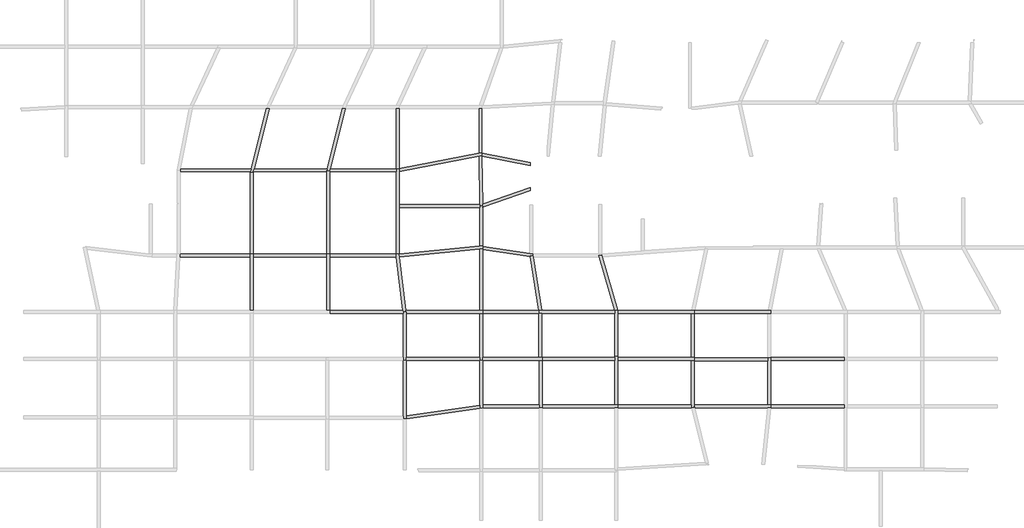
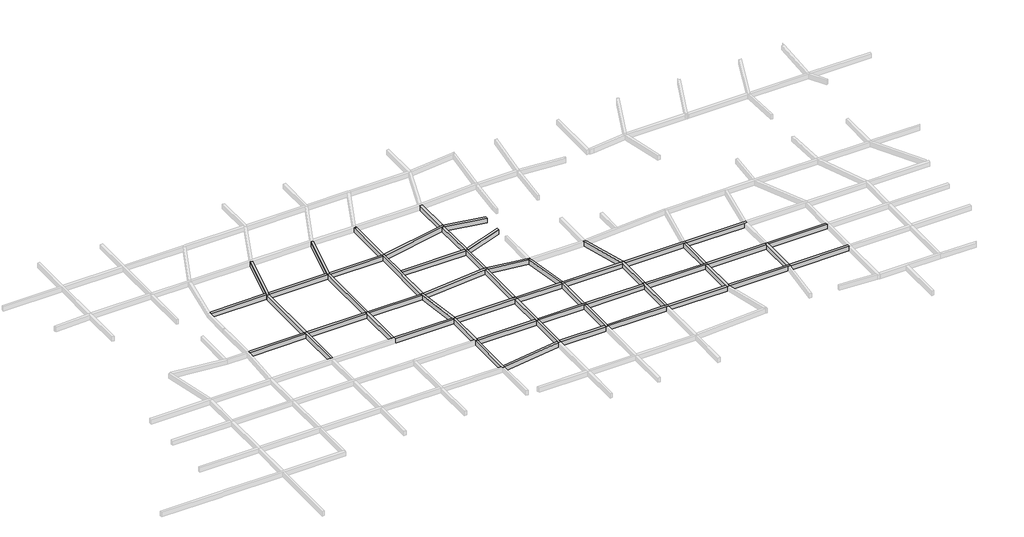
# One storey, part 5 of 15: 56 beams.
"""IFC4 building model written with IfcOpenShell, lengths in millimetres."""

from ifc_helpers import new_model, si_unit, frame, origin, place, context, project, spatial, polyline, outline, extrude, faceted_brep, element, save

model = new_model("IFC4")

# Units and contexts
model_context = context("Model", 3, world=origin())
ifc_project = project(units=[si_unit("LENGTHUNIT", "METRE", prefix="MILLI")], contexts=[model_context])

# Site, building, storey
site = spatial("IfcSite", under=ifc_project)
building = spatial("IfcBuilding", under=site)
storey = spatial("IfcBuildingStorey", under=building, Name="层高", Elevation=3300.0)

# Beams
placement = place(None, origin())
element("IfcBeam", 1, ObjectType="混凝土 - 矩形梁 : KL_beam", at=placement, inside=storey, context=model_context, shape_type="Brep", body=[
    faceted_brep([(196149.7804968, 49107.4754781, 3300.0), (195849.7804968, 49107.4754781, 3300.0), (195849.7804968, 48807.4754781, 3300.0), (195849.7804968, 43342.2492414, 3300.0), (196149.7804968, 43342.2492414, 3300.0), (196149.7804968, 48807.4754781, 3300.0), (196149.7804968, 49107.4754781, 2700.0), (196149.7804968, 43342.2492414, 2700.0), (196149.7804968, 48807.4754781, 2700.0), (195849.7804968, 49107.4754781, 2700.0), (195849.7804968, 43342.2492414, 2700.0), (195849.7804968, 48807.4754781, 2700.0)], [[[0, 1, 2, 3, 4, 5]], [[6, 0, 5, 4, 7, 8]], [[9, 6, 8, 7, 10, 11]], [[1, 9, 11, 10, 3, 2]], [[4, 3, 10, 7]], [[1, 0, 6, 9]]]),
])
element("IfcBeam", 2, ObjectType="混凝土 - 矩形梁 : KL_beam", at=placement, inside=storey, context=model_context, shape_type="Brep", body=[
    faceted_brep([(203965.7079926, 49107.4754781, 3300.0), (203665.7079926, 49107.4754781, 3300.0), (203665.7079926, 48807.4754781, 3300.0), (203665.7079926, 43342.2492414, 3300.0), (203965.7079926, 43342.2492414, 3300.0), (203965.7079926, 48807.4754781, 3300.0), (203965.7079926, 49107.4754781, 2700.0), (203965.7079926, 43342.2492414, 2700.0), (203965.7079926, 48807.4754781, 2700.0), (203665.7079926, 49107.4754781, 2700.0), (203665.7079926, 43342.2492414, 2700.0), (203665.7079926, 48807.4754781, 2700.0)], [[[0, 1, 2, 3, 4, 5]], [[6, 0, 5, 4, 7, 8]], [[9, 6, 8, 7, 10, 11]], [[1, 9, 11, 10, 3, 2]], [[4, 3, 10, 7]], [[1, 0, 6, 9]]]),
])
element("IfcBeam", 3, ObjectType="混凝土 - 矩形梁 : KL_beam", at=placement, inside=storey, context=model_context, shape_type="Brep", body=[
    faceted_brep([(211749.7804968, 43201.435443, 3300.0), (211449.7804968, 43183.086657, 3300.0), (211449.7804968, 43042.2492414, 3300.0), (211449.7804968, 38542.26105, 3300.0), (211449.7804968, 38242.26105, 3300.0), (211749.7804968, 38242.26105, 3300.0), (211749.7804968, 38539.4462664, 3300.0), (211749.7804968, 43039.4462664, 3300.0), (211449.7804968, 43183.086657, 2700.0), (211449.7804968, 43042.2492414, 2700.0), (211449.7804968, 38542.26105, 2700.0), (211449.7804968, 38242.26105, 2700.0), (211749.7804968, 43201.435443, 2700.0), (211749.7804968, 43039.4462664, 2700.0), (211749.7804968, 38539.4462664, 2700.0), (211749.7804968, 38242.26105, 2700.0)], [[[0, 1, 2, 3, 4, 5, 6, 7]], [[1, 8, 9, 10, 11, 4, 3, 2]], [[8, 12, 13, 14, 15, 11, 10, 9]], [[12, 0, 7, 6, 5, 15, 14, 13]], [[5, 4, 11, 15]], [[0, 12, 8, 1]]]),
])
element("IfcBeam", 4, ObjectType="混凝土 - 矩形梁 : KL_beam", at=placement, inside=storey, context=model_context, shape_type="Brep", body=[
    faceted_brep([(211449.7804968, 32262.7548984, 3300.0), (211749.7804968, 32262.7548984, 3300.0), (211749.7804968, 32565.9979708, 3300.0), (211749.7804968, 38239.4462664, 3300.0), (211749.7804968, 38242.26105, 3300.0), (211449.7804968, 38242.26105, 3300.0), (211449.7804968, 32542.26105, 3300.0), (211449.7804968, 32262.7548984, 2700.0), (211449.7804968, 38242.26105, 2700.0), (211449.7804968, 32542.26105, 2700.0), (211749.7804968, 32262.7548984, 2700.0), (211749.7804968, 38242.26105, 2700.0), (211749.7804968, 38239.4462664, 2700.0), (211749.7804968, 32565.9979708, 2700.0)], [[[0, 1, 2, 3, 4, 5, 6]], [[7, 0, 6, 5, 8, 9]], [[10, 7, 9, 8, 11, 12, 13]], [[1, 10, 13, 12, 11, 4, 3, 2]], [[5, 4, 11, 8]], [[1, 0, 7, 10]]]),
])
element("IfcBeam", 5, ObjectType="混凝土 - 矩形梁 : KL_beam", at=placement, inside=storey, context=model_context, shape_type="Brep", body=[
    faceted_brep([(210725.2131667, 49084.2140037, 3300.0), (210759.1923851, 48807.4754781, 3300.0), (211430.2377888, 43342.2492414, 3300.0), (211449.7804968, 43183.086657, 3300.0), (211749.7804968, 43201.435443, 3300.0), (211732.8348985, 43339.4462664, 3300.0), (211059.55045, 48822.9080592, 3300.0), (211022.9770122, 49120.7748067, 3300.0), (211749.7804968, 43201.435443, 2700.0), (211732.8348985, 43339.4462664, 2700.0), (211059.55045, 48822.9080592, 2700.0), (211022.9770122, 49120.7748067, 2700.0), (211449.7804968, 43183.086657, 2700.0), (211430.2377888, 43342.2492414, 2700.0), (210759.1923851, 48807.4754781, 2700.0), (210725.2131667, 49084.2140037, 2700.0)], [[[0, 1, 2, 3, 4, 5, 6, 7]], [[7, 6, 5, 4, 8, 9, 10, 11]], [[11, 10, 9, 8, 12, 13, 14, 15]], [[3, 2, 1, 0, 15, 14, 13, 12]], [[3, 12, 8, 4]], [[0, 7, 11, 15]]]),
])
element("IfcBeam", 6, ObjectType="混凝土 - 矩形梁 : KL_beam", at=placement, inside=storey, context=model_context, shape_type="SweptSolid", body=[
    extrude(outline(polyline([(203965.7079926, 43042.2492414), (203965.7079926, 43342.2492414), (211430.2377888, 43342.2492414), (211449.7804968, 43183.086657), (211449.7804968, 43042.2492414), (203965.7079926, 43042.2492414)])), frame((0.0, 0.0, 2700.0), z_axis=(0.0, 0.0, 1.0), x_axis=(1.0, 0.0, 0.0)), (0.0, 0.0, 1.0), 600.0),
])
element("IfcBeam", 7, ObjectType="混凝土 - 矩形梁 : KL_beam", at=placement, inside=storey, context=model_context, shape_type="Brep", body=[
    faceted_brep([(211732.8348985, 43339.4462664, 3300.0), (211749.7804968, 43201.435443, 3300.0), (211749.7804968, 43042.2492414, 3300.0), (211749.7804968, 43039.4462664, 3300.0), (219249.7804968, 43039.4462664, 3300.0), (219549.7804968, 43039.4462664, 3300.0), (219549.7804968, 43042.26105, 3300.0), (219549.7804968, 43339.4462664, 3300.0), (219249.7804968, 43339.4462664, 3300.0), (211749.7804968, 43039.4462664, 2700.0), (219249.7804968, 43039.4462664, 2700.0), (219549.7804968, 43039.4462664, 2700.0), (211749.7804968, 43201.435443, 2700.0), (211732.8348985, 43339.4462664, 2700.0), (219249.7804968, 43339.4462664, 2700.0), (219549.7804968, 43339.4462664, 2700.0), (219549.7804968, 43042.26105, 2700.0), (211749.7804968, 43042.2492414, 2700.0)], [[[0, 1, 2, 3, 4, 5, 6, 7, 8]], [[3, 9, 10, 11, 5, 4]], [[12, 13, 14, 15, 16, 11, 10, 9, 17]], [[13, 0, 8, 7, 15, 14]], [[9, 3, 2, 1, 12, 17]], [[1, 0, 13, 12]], [[7, 6, 5, 11, 16, 15]]]),
])
element("IfcBeam", 8, ObjectType="混凝土 - 矩形梁 : KL_beam", at=placement, inside=storey, context=model_context, shape_type="Brep", body=[
    faceted_brep([(219249.7804968, 38239.4462664, 3300.0), (219549.7804968, 38239.4462664, 3300.0), (219549.7804968, 38539.4462664, 3300.0), (219549.7804968, 43039.4462664, 3300.0), (219249.7804968, 43039.4462664, 3300.0), (219249.7804968, 38539.4462664, 3300.0), (219249.7804968, 38239.4462664, 2700.0), (219249.7804968, 43039.4462664, 2700.0), (219249.7804968, 38539.4462664, 2700.0), (219549.7804968, 38239.4462664, 2700.0), (219549.7804968, 43039.4462664, 2700.0), (219549.7804968, 38539.4462664, 2700.0)], [[[0, 1, 2, 3, 4, 5]], [[6, 0, 5, 4, 7, 8]], [[9, 6, 8, 7, 10, 11]], [[1, 9, 11, 10, 3, 2]], [[4, 3, 10, 7]], [[1, 0, 6, 9]]]),
])
element("IfcBeam", 9, ObjectType="混凝土 - 矩形梁 : KL_beam", at=placement, inside=storey, context=model_context, shape_type="Brep", body=[
    faceted_brep([(211749.7804968, 38539.4462664, 3300.0), (211749.7804968, 38242.26105, 3300.0), (211749.7804968, 38239.4462664, 3300.0), (219249.7804968, 38239.4462664, 3300.0), (219249.7804968, 38539.4462664, 3300.0), (211749.7804968, 38539.4462664, 2700.0), (219249.7804968, 38539.4462664, 2700.0), (211749.7804968, 38239.4462664, 2700.0), (211749.7804968, 38242.26105, 2700.0), (219249.7804968, 38239.4462664, 2700.0)], [[[0, 1, 2, 3, 4]], [[5, 0, 4, 6]], [[7, 8, 5, 6, 9]], [[2, 7, 9, 3]], [[0, 5, 8, 7, 2, 1]], [[4, 3, 9, 6]]]),
])
element("IfcBeam", 10, ObjectType="混凝土 - 矩形梁 : KL_beam", at=placement, inside=storey, context=model_context, shape_type="Brep", body=[
    faceted_brep([(219249.7804968, 33368.5241292, 3300.0), (219549.7804968, 33412.7548984, 3300.0), (219549.7804968, 33692.26105, 3300.0), (219549.7804968, 38239.4462664, 3300.0), (219249.7804968, 38239.4462664, 3300.0), (219249.7804968, 33671.7672016, 3300.0), (219249.7804968, 33368.5241292, 2700.0), (219249.7804968, 38239.4462664, 2700.0), (219249.7804968, 33671.7672016, 2700.0), (219549.7804968, 33412.7548984, 2700.0), (219549.7804968, 38239.4462664, 2700.0), (219549.7804968, 33692.26105, 2700.0)], [[[0, 1, 2, 3, 4, 5]], [[6, 0, 5, 4, 7, 8]], [[9, 6, 8, 7, 10, 11]], [[1, 9, 11, 10, 3, 2]], [[4, 3, 10, 7]], [[1, 0, 6, 9]]]),
])
element("IfcBeam", 11, ObjectType="混凝土 - 矩形梁 : KL_beam", at=placement, inside=storey, context=model_context, shape_type="SweptSolid", body=[
    extrude(outline(polyline([(211749.7804968, 32262.7548984), (211749.7804968, 32565.9979708), (219249.7804968, 33671.7672016), (219249.7804968, 33368.5241292), (211749.7804968, 32262.7548984)])), frame((0.0, 0.0, 2700.0), z_axis=(0.0, 0.0, 1.0), x_axis=(1.0, 0.0, 0.0)), (0.0, 0.0, 1.0), 600.0),
])
element("IfcBeam", 12, ObjectType="混凝土 - 矩形梁 : KL_beam", at=placement, inside=storey, context=model_context, shape_type="Brep", body=[
    faceted_brep([(225649.7804968, 38239.4462664, 3300.0), (225649.7804968, 38539.4462664, 3300.0), (225589.7804968, 38539.4462664, 3300.0), (225289.7804968, 38539.4462664, 3300.0), (219549.7804968, 38539.4462664, 3300.0), (219549.7804968, 38239.4462664, 3300.0), (225349.7804968, 38239.4462664, 3300.0), (225649.7804968, 38239.4462664, 2700.0), (219549.7804968, 38239.4462664, 2700.0), (225349.7804968, 38239.4462664, 2700.0), (225649.7804968, 38539.4462664, 2700.0), (219549.7804968, 38539.4462664, 2700.0), (225289.7804968, 38539.4462664, 2700.0), (225589.7804968, 38539.4462664, 2700.0)], [[[0, 1, 2, 3, 4, 5, 6]], [[7, 0, 6, 5, 8, 9]], [[10, 7, 9, 8, 11, 12, 13]], [[1, 10, 13, 12, 11, 4, 3, 2]], [[5, 4, 11, 8]], [[1, 0, 7, 10]]]),
])
element("IfcBeam", 13, ObjectType="混凝土 - 矩形梁 : KL_beam", at=placement, inside=storey, context=model_context, shape_type="Brep", body=[
    faceted_brep([(225349.7804968, 33392.26105, 3300.0), (225649.7804968, 33392.26105, 3300.0), (225649.7804968, 33692.26105, 3300.0), (225649.7804968, 38239.4462664, 3300.0), (225349.7804968, 38239.4462664, 3300.0), (225349.7804968, 33692.26105, 3300.0), (225349.7804968, 33392.26105, 2700.0), (225349.7804968, 38239.4462664, 2700.0), (225349.7804968, 33692.26105, 2700.0), (225649.7804968, 33392.26105, 2700.0), (225649.7804968, 38239.4462664, 2700.0), (225649.7804968, 33692.26105, 2700.0)], [[[0, 1, 2, 3, 4, 5]], [[6, 0, 5, 4, 7, 8]], [[9, 6, 8, 7, 10, 11]], [[1, 9, 11, 10, 3, 2]], [[4, 3, 10, 7]], [[1, 0, 6, 9]]]),
])
element("IfcBeam", 14, ObjectType="混凝土 - 矩形梁 : KL_beam", at=placement, inside=storey, context=model_context, shape_type="Brep", body=[
    faceted_brep([(219549.7804968, 33692.26105, 3300.0), (219549.7804968, 33412.7548984, 3300.0), (219549.7804968, 33392.26105, 3300.0), (225349.7804968, 33392.26105, 3300.0), (225349.7804968, 33692.26105, 3300.0), (219549.7804968, 33392.26105, 2700.0), (225349.7804968, 33392.26105, 2700.0), (219549.7804968, 33412.7548984, 2700.0), (219549.7804968, 33692.26105, 2700.0), (225349.7804968, 33692.26105, 2700.0)], [[[0, 1, 2, 3, 4]], [[2, 5, 6, 3]], [[5, 7, 8, 9, 6]], [[8, 0, 4, 9]], [[0, 8, 7, 5, 2, 1]], [[4, 3, 6, 9]]]),
])
element("IfcBeam", 15, ObjectType="混凝土 - 矩形梁 : KL_beam", at=placement, inside=storey, context=model_context, shape_type="Brep", body=[
    faceted_brep([(233349.8189959, 33392.26105, 3300.0), (233349.8189959, 33692.26105, 3300.0), (233049.8189959, 33692.26105, 3300.0), (225649.7804968, 33692.26105, 3300.0), (225649.7804968, 33392.26105, 3300.0), (233049.8189959, 33392.26105, 3300.0), (233349.8189959, 33392.26105, 2700.0), (225649.7804968, 33392.26105, 2700.0), (233049.8189959, 33392.26105, 2700.0), (233349.8189959, 33692.26105, 2700.0), (225649.7804968, 33692.26105, 2700.0), (233049.8189959, 33692.26105, 2700.0)], [[[0, 1, 2, 3, 4, 5]], [[6, 0, 5, 4, 7, 8]], [[9, 6, 8, 7, 10, 11]], [[1, 9, 11, 10, 3, 2]], [[4, 3, 10, 7]], [[1, 0, 6, 9]]]),
])
element("IfcBeam", 16, ObjectType="混凝土 - 矩形梁 : KL_beam", at=placement, inside=storey, context=model_context, shape_type="Brep", body=[
    faceted_brep([(233049.8189959, 38642.26105, 3300.0), (233349.8189959, 38642.26105, 3300.0), (233349.8189959, 38642.26105, 2700.0), (233049.8189959, 38642.26105, 2700.0), (233049.8189959, 38539.4462664, 3300.0), (233049.8189959, 38239.4462664, 3300.0), (233049.8189959, 33692.26105, 3300.0), (233349.8189959, 33692.26105, 3300.0), (233349.8189959, 38239.4462664, 3300.0), (233349.8189959, 38539.4462664, 3300.0), (233349.8189959, 33692.26105, 2700.0), (233349.8189959, 38239.4462664, 2700.0), (233349.8189959, 38539.4462664, 2700.0), (233049.8189959, 33692.26105, 2700.0), (233049.8189959, 38239.4462664, 2700.0), (233049.8189959, 38539.4462664, 2700.0)], [[[0, 1, 2, 3]], [[1, 0, 4, 5, 6, 7, 8, 9]], [[2, 1, 9, 8, 7, 10, 11, 12]], [[3, 2, 12, 11, 10, 13, 14, 15]], [[0, 3, 15, 14, 13, 6, 5, 4]], [[7, 6, 13, 10]]]),
])
element("IfcBeam", 17, ObjectType="混凝土 - 矩形梁 : KL_beam", at=placement, inside=storey, context=model_context, shape_type="SweptSolid", body=[
    extrude(outline(polyline([(225649.7804968, 38239.4462664), (225649.7804968, 38539.4462664), (233049.8189959, 38539.4462664), (233049.8189959, 38239.4462664), (225649.7804968, 38239.4462664)])), frame((0.0, 0.0, 2700.0), z_axis=(0.0, 0.0, 1.0), x_axis=(1.0, 0.0, 0.0)), (0.0, 0.0, 1.0), 600.0),
])
element("IfcBeam", 18, ObjectType="混凝土 - 矩形梁 : KL_beam", at=placement, inside=storey, context=model_context, shape_type="Brep", body=[
    faceted_brep([(233349.8189959, 43342.26105, 3300.0), (233312.8521034, 43342.26105, 3300.0), (233049.8189959, 43342.26105, 3300.0), (233049.8189959, 43042.26105, 3300.0), (233049.8189959, 38642.26105, 3300.0), (233349.8189959, 38642.26105, 3300.0), (233349.8189959, 43042.26105, 3300.0), (233349.8189959, 43342.26105, 2700.0), (233349.8189959, 38642.26105, 2700.0), (233349.8189959, 43042.26105, 2700.0), (233049.8189959, 43342.26105, 2700.0), (233312.8521034, 43342.26105, 2700.0), (233049.8189959, 38642.26105, 2700.0), (233049.8189959, 43042.26105, 2700.0)], [[[0, 1, 2, 3, 4, 5, 6]], [[7, 0, 6, 5, 8, 9]], [[10, 11, 7, 9, 8, 12, 13]], [[2, 10, 13, 12, 4, 3]], [[5, 4, 12, 8]], [[2, 1, 0, 7, 11, 10]]]),
])
element("IfcBeam", 19, ObjectType="混凝土 - 矩形梁 : KL_beam", at=placement, inside=storey, context=model_context, shape_type="Brep", body=[
    faceted_brep([(225289.7804968, 43342.26105, 3300.0), (225289.7804968, 43042.26105, 3300.0), (225589.7804968, 43042.26105, 3300.0), (233049.8189959, 43042.26105, 3300.0), (233049.8189959, 43342.26105, 3300.0), (233000.7622727, 43342.26105, 3300.0), (225567.8925996, 43342.26105, 3300.0), (225289.7804968, 43342.26105, 2700.0), (233049.8189959, 43342.26105, 2700.0), (233000.7622727, 43342.26105, 2700.0), (225567.8925996, 43342.26105, 2700.0), (225289.7804968, 43042.26105, 2700.0), (233049.8189959, 43042.26105, 2700.0), (225589.7804968, 43042.26105, 2700.0)], [[[0, 1, 2, 3, 4, 5, 6]], [[7, 0, 6, 5, 4, 8, 9, 10]], [[11, 7, 10, 9, 8, 12, 13]], [[1, 11, 13, 12, 3, 2]], [[4, 3, 12, 8]], [[1, 0, 7, 11]]]),
])
element("IfcBeam", 20, ObjectType="混凝土 - 矩形梁 : KL_beam", at=placement, inside=storey, context=model_context, shape_type="SweptSolid", body=[
    extrude(outline(polyline([(225589.7804968, 38539.4462664), (225289.7804968, 38539.4462664), (225289.7804968, 43042.26105), (225589.7804968, 43042.26105), (225589.7804968, 38539.4462664)])), frame((0.0, 0.0, 2700.0), z_axis=(0.0, 0.0, 1.0), x_axis=(1.0, 0.0, 0.0)), (0.0, 0.0, 1.0), 600.0),
])
element("IfcBeam", 21, ObjectType="混凝土 - 矩形梁 : KL_beam", at=placement, inside=storey, context=model_context, shape_type="Brep", body=[
    faceted_brep([(219249.7804968, 43342.26105, 3300.0), (219249.7804968, 43339.4462664, 3300.0), (219549.7804968, 43339.4462664, 3300.0), (219549.7804968, 43042.26105, 3300.0), (225289.7804968, 43042.26105, 3300.0), (225289.7804968, 43342.26105, 3300.0), (225264.1530619, 43342.26105, 3300.0), (219549.7804968, 43342.26105, 3300.0), (219249.7804968, 43342.26105, 2700.0), (225289.7804968, 43342.26105, 2700.0), (225264.1530619, 43342.26105, 2700.0), (219549.7804968, 43342.26105, 2700.0), (219249.7804968, 43339.4462664, 2700.0), (225289.7804968, 43042.26105, 2700.0), (219549.7804968, 43042.26105, 2700.0), (219549.7804968, 43339.4462664, 2700.0)], [[[0, 1, 2, 3, 4, 5, 6, 7]], [[8, 0, 7, 6, 5, 9, 10, 11]], [[12, 8, 11, 10, 9, 13, 14, 15]], [[3, 14, 13, 4]], [[0, 8, 12, 1]], [[15, 2, 1, 12]], [[2, 15, 14, 3]], [[5, 4, 13, 9]]]),
])
element("IfcBeam", 22, ObjectType="混凝土 - 矩形梁 : KL_beam", at=placement, inside=storey, context=model_context, shape_type="Brep", body=[
    faceted_brep([(241149.8189959, 38239.4462664, 3300.0), (241149.8189959, 38517.26105, 3300.0), (241149.8189959, 38539.4462664, 3300.0), (240849.8189959, 38539.4462664, 3300.0), (233349.8189959, 38539.4462664, 3300.0), (233349.8189959, 38239.4462664, 3300.0), (240849.8189959, 38239.4462664, 3300.0), (241149.8189959, 38239.4462664, 2700.0), (233349.8189959, 38239.4462664, 2700.0), (240849.8189959, 38239.4462664, 2700.0), (241149.8189959, 38539.4462664, 2700.0), (241149.8189959, 38517.26105, 2700.0), (233349.8189959, 38539.4462664, 2700.0), (240849.8189959, 38539.4462664, 2700.0)], [[[0, 1, 2, 3, 4, 5, 6]], [[7, 0, 6, 5, 8, 9]], [[10, 11, 7, 9, 8, 12, 13]], [[2, 10, 13, 12, 4, 3]], [[5, 4, 12, 8]], [[2, 1, 0, 7, 11, 10]]]),
])
element("IfcBeam", 23, ObjectType="混凝土 - 矩形梁 : KL_beam", at=placement, inside=storey, context=model_context, shape_type="Brep", body=[
    faceted_brep([(240849.8189959, 33392.26105, 3300.0), (240882.0776299, 33392.26105, 3300.0), (241149.8189959, 33392.26105, 3300.0), (241149.8189959, 33560.3336966, 3300.0), (241149.8189959, 33692.26105, 3300.0), (241149.8189959, 38217.26105, 3300.0), (241149.8189959, 38239.4462664, 3300.0), (240849.8189959, 38239.4462664, 3300.0), (240849.8189959, 33692.26105, 3300.0), (241149.8189959, 33392.26105, 2700.0), (241149.8189959, 33560.3336966, 2700.0), (241149.8189959, 33692.26105, 2700.0), (241149.8189959, 38217.26105, 2700.0), (241149.8189959, 38239.4462664, 2700.0), (240882.0776299, 33392.26105, 2700.0), (240849.8189959, 33392.26105, 2700.0), (240849.8189959, 33692.26105, 2700.0), (240849.8189959, 38239.4462664, 2700.0)], [[[0, 1, 2, 3, 4, 5, 6, 7, 8]], [[2, 9, 10, 11, 12, 13, 6, 5, 4, 3]], [[9, 14, 15, 16, 17, 13, 12, 11, 10]], [[15, 0, 8, 7, 17, 16]], [[7, 6, 13, 17]], [[2, 1, 0, 15, 14, 9]]]),
])
element("IfcBeam", 24, ObjectType="混凝土 - 矩形梁 : KL_beam", at=placement, inside=storey, context=model_context, shape_type="SweptSolid", body=[
    extrude(outline(polyline([(233349.8189959, 33392.26105), (233349.8189959, 33692.26105), (240849.8189959, 33692.26105), (240849.8189959, 33392.26105), (233349.8189959, 33392.26105)])), frame((0.0, 0.0, 2700.0), z_axis=(0.0, 0.0, 1.0), x_axis=(1.0, 0.0, 0.0)), (0.0, 0.0, 1.0), 600.0),
])
element("IfcBeam", 25, ObjectType="混凝土 - 矩形梁 : KL_beam", at=placement, inside=storey, context=model_context, shape_type="Brep", body=[
    faceted_brep([(233349.8189959, 43042.26105, 3300.0), (233349.8189959, 43042.26105, 2700.0), (240849.8189959, 43042.26105, 2700.0), (241149.8189959, 43042.26105, 2700.0), (241149.8189959, 43042.26105, 3300.0), (240849.8189959, 43042.26105, 3300.0), (233349.8189959, 43342.26105, 3300.0), (233349.8189959, 43342.26105, 2700.0), (241149.8189959, 43342.26105, 3300.0), (241149.8189959, 43342.26105, 2700.0), (240878.4550975, 43342.26105, 3300.0), (240878.4550975, 43342.26105, 2700.0)], [[[0, 1, 2, 3, 4, 5]], [[0, 6, 7, 1]], [[8, 4, 3, 9]], [[6, 0, 5, 4, 8, 10]], [[1, 7, 11, 9, 3, 2]], [[7, 6, 10, 8, 9, 11]]]),
])
element("IfcBeam", 26, ObjectType="混凝土 - 矩形梁 : KL_beam", at=placement, inside=storey, context=model_context, shape_type="SweptSolid", body=[
    extrude(outline(polyline([(241149.8189959, 38539.4462664), (240849.8189959, 38539.4462664), (240849.8189959, 43042.26105), (241149.8189959, 43042.26105), (241149.8189959, 38539.4462664)])), frame((0.0, 0.0, 2700.0), z_axis=(0.0, 0.0, 1.0), x_axis=(1.0, 0.0, 0.0)), (0.0, 0.0, 1.0), 600.0),
])
element("IfcBeam", 27, ObjectType="混凝土 - 矩形梁 : KL_beam", at=placement, inside=storey, context=model_context, shape_type="Brep", body=[
    faceted_brep([(248949.8189959, 33392.26105, 3300.0), (248949.8189959, 33692.26105, 3300.0), (248649.8189959, 33692.26105, 3300.0), (241149.8189959, 33692.26105, 3300.0), (241149.8189959, 33560.3336966, 3300.0), (241190.9158106, 33392.26105, 3300.0), (248633.2271187, 33392.26105, 3300.0), (248934.8796026, 33392.26105, 3300.0), (248949.8189959, 33392.26105, 2700.0), (241190.9158106, 33392.26105, 2700.0), (248633.2271187, 33392.26105, 2700.0), (248934.8796026, 33392.26105, 2700.0), (248949.8189959, 33692.26105, 2700.0), (241149.8189959, 33560.3336966, 2700.0), (241149.8189959, 33692.26105, 2700.0), (248649.8189959, 33692.26105, 2700.0)], [[[0, 1, 2, 3, 4, 5, 6, 7]], [[8, 0, 7, 6, 5, 9, 10, 11]], [[12, 8, 11, 10, 9, 13, 14, 15]], [[14, 3, 2, 1, 12, 15]], [[3, 14, 13, 4]], [[5, 4, 13, 9]], [[1, 0, 8, 12]]]),
])
element("IfcBeam", 28, ObjectType="混凝土 - 矩形梁 : KL_beam", at=placement, inside=storey, context=model_context, shape_type="Brep", body=[
    faceted_brep([(248949.8189959, 38517.26105, 3300.0), (248649.8189959, 38517.26105, 3300.0), (248649.8189959, 38217.26105, 3300.0), (248649.8189959, 33692.26105, 3300.0), (248949.8189959, 33692.26105, 3300.0), (248949.8189959, 38242.26105, 3300.0), (248649.8189959, 38517.26105, 2700.0), (248649.8189959, 38217.26105, 2700.0), (248649.8189959, 33692.26105, 2700.0), (248949.8189959, 38517.26105, 2700.0), (248949.8189959, 38242.26105, 2700.0), (248949.8189959, 33692.26105, 2700.0)], [[[0, 1, 2, 3, 4, 5]], [[1, 6, 7, 8, 3, 2]], [[6, 9, 10, 11, 8, 7]], [[9, 0, 5, 4, 11, 10]], [[4, 3, 8, 11]], [[1, 0, 9, 6]]]),
])
element("IfcBeam", 29, ObjectType="混凝土 - 矩形梁 : KL_beam", at=placement, inside=storey, context=model_context, shape_type="Brep", body=[
    faceted_brep([(241149.8189959, 38517.26105, 3300.0), (241149.8189959, 38239.4462664, 3300.0), (241149.8189959, 38217.26105, 3300.0), (248649.8189959, 38217.26105, 3300.0), (248649.8189959, 38517.26105, 3300.0), (241149.8189959, 38517.26105, 2700.0), (248649.8189959, 38517.26105, 2700.0), (241149.8189959, 38217.26105, 2700.0), (241149.8189959, 38239.4462664, 2700.0), (248649.8189959, 38217.26105, 2700.0)], [[[0, 1, 2, 3, 4]], [[5, 0, 4, 6]], [[7, 8, 5, 6, 9]], [[2, 7, 9, 3]], [[0, 5, 8, 7, 2, 1]], [[4, 3, 9, 6]]]),
])
element("IfcBeam", 30, ObjectType="混凝土 - 矩形梁 : KL_beam", at=placement, inside=storey, context=model_context, shape_type="Brep", body=[
    faceted_brep([(248949.8189959, 43042.26105, 3300.0), (248949.8189959, 43342.26105, 3300.0), (248676.168538, 43342.26105, 3300.0), (241185.211854, 43342.26105, 3300.0), (241149.8189959, 43342.26105, 3300.0), (241149.8189959, 43042.26105, 3300.0), (248649.8189959, 43042.26105, 3300.0), (248949.8189959, 43042.26105, 2700.0), (241149.8189959, 43042.26105, 2700.0), (248649.8189959, 43042.26105, 2700.0), (248949.8189959, 43342.26105, 2700.0), (241149.8189959, 43342.26105, 2700.0), (241185.211854, 43342.26105, 2700.0), (248676.168538, 43342.26105, 2700.0)], [[[0, 1, 2, 3, 4, 5, 6]], [[7, 0, 6, 5, 8, 9]], [[10, 7, 9, 8, 11, 12, 13]], [[1, 10, 13, 12, 11, 4, 3, 2]], [[5, 4, 11, 8]], [[1, 0, 7, 10]]]),
])
element("IfcBeam", 31, ObjectType="混凝土 - 矩形梁 : KL_beam", at=placement, inside=storey, context=model_context, shape_type="Brep", body=[
    faceted_brep([(248949.8189959, 38542.26105, 3300.0), (248949.8189959, 38517.26105, 3300.0), (248949.8189959, 38242.26105, 3300.0), (256449.8189959, 38242.26105, 3300.0), (256449.8189959, 38542.26105, 3300.0), (248949.8189959, 38542.26105, 2700.0), (256449.8189959, 38542.26105, 2700.0), (248949.8189959, 38242.26105, 2700.0), (248949.8189959, 38517.26105, 2700.0), (256449.8189959, 38242.26105, 2700.0)], [[[0, 1, 2, 3, 4]], [[5, 0, 4, 6]], [[7, 8, 5, 6, 9]], [[2, 7, 9, 3]], [[7, 2, 1, 0, 5, 8]], [[4, 3, 9, 6]]]),
])
element("IfcBeam", 32, ObjectType="混凝土 - 矩形梁 : KL_beam", at=placement, inside=storey, context=model_context, shape_type="Brep", body=[
    faceted_brep([(248949.8189959, 33692.26105, 3300.0), (248949.8189959, 33392.26105, 3300.0), (256405.4878315, 33392.26105, 3300.0), (256449.8189959, 33392.26105, 3300.0), (256449.8189959, 33692.26105, 3300.0), (248949.8189959, 33692.26105, 2700.0), (256449.8189959, 33692.26105, 2700.0), (248949.8189959, 33392.26105, 2700.0), (256449.8189959, 33392.26105, 2700.0), (256405.4878315, 33392.26105, 2700.0)], [[[0, 1, 2, 3, 4]], [[5, 0, 4, 6]], [[7, 5, 6, 8, 9]], [[1, 7, 9, 8, 3, 2]], [[1, 0, 5, 7]], [[4, 3, 8, 6]]]),
])
element("IfcBeam", 33, ObjectType="混凝土 - 矩形梁 : KL_beam", at=placement, inside=storey, context=model_context, shape_type="Brep", body=[
    faceted_brep([(233312.8521034, 43342.26105, 3300.0), (231741.7485438, 48821.3502966, 3300.0), (231696.6703608, 48978.5566033, 3300.0), (231396.6703608, 48936.3943529, 3300.0), (231433.6372532, 48807.4754781, 3300.0), (233000.7622727, 43342.26105, 3300.0), (233049.8189959, 43342.26105, 3300.0), (233312.8521034, 43342.26105, 2700.0), (231741.7485438, 48821.3502966, 2700.0), (231696.6703608, 48978.5566033, 2700.0), (233049.8189959, 43342.26105, 2700.0), (233000.7622727, 43342.26105, 2700.0), (231433.6372532, 48807.4754781, 2700.0), (231396.6703608, 48936.3943529, 2700.0)], [[[0, 1, 2, 3, 4, 5, 6]], [[2, 1, 0, 7, 8, 9]], [[9, 8, 7, 10, 11, 12, 13]], [[5, 4, 3, 13, 12, 11]], [[7, 0, 6, 5, 11, 10]], [[3, 2, 9, 13]]]),
])
element("IfcBeam", 34, ObjectType="混凝土 - 矩形梁 : KL_beam", at=placement, inside=storey, context=model_context, shape_type="Brep", body=[
    faceted_brep([(225264.1530619, 43342.26105, 3300.0), (225289.7804968, 43342.26105, 3300.0), (225567.8925996, 43342.26105, 3300.0), (224702.2876712, 48807.4754781, 3300.0), (224676.6602363, 48969.2807341, 3300.0), (224376.6602363, 48945.6702221, 3300.0), (224395.616179, 48825.9871097, 3300.0), (225567.8925996, 43342.26105, 2700.0), (224702.2876712, 48807.4754781, 2700.0), (224676.6602363, 48969.2807341, 2700.0), (225289.7804968, 43342.26105, 2700.0), (225264.1530619, 43342.26105, 2700.0), (224395.616179, 48825.9871097, 2700.0), (224376.6602363, 48945.6702221, 2700.0)], [[[0, 1, 2, 3, 4, 5, 6]], [[4, 3, 2, 7, 8, 9]], [[9, 8, 7, 10, 11, 12, 13]], [[5, 13, 12, 11, 0, 6]], [[0, 11, 10, 7, 2, 1]], [[5, 4, 9, 13]]]),
])
element("IfcBeam", 35, ObjectType="混凝土 - 矩形梁 : KL_beam", at=placement, inside=storey, context=model_context, shape_type="Brep", body=[
    faceted_brep([(219549.7804968, 49639.5134023, 3300.0), (219549.7804968, 49880.2658789, 3300.0), (219549.7804968, 49940.8978477, 3300.0), (219249.7804968, 49912.0433171, 3300.0), (211041.9011747, 49122.5949661, 3300.0), (211022.9770122, 49120.7748067, 3300.0), (211059.55045, 48822.9080592, 3300.0), (219249.7804968, 49610.6588717, 3300.0), (219549.7804968, 49639.5134023, 2700.0), (211059.55045, 48822.9080592, 2700.0), (219249.7804968, 49610.6588717, 2700.0), (219549.7804968, 49940.8978477, 2700.0), (219549.7804968, 49880.2658789, 2700.0), (211022.9770122, 49120.7748067, 2700.0), (211041.9011747, 49122.5949661, 2700.0), (219249.7804968, 49912.0433171, 2700.0), (210724.2518995, 49092.042897, 2700.0), (210724.2518995, 49092.042897, 3300.0), (210884.7041486, 49107.4754781, 3300.0), (210884.7041486, 49107.4754781, 2700.0), (210725.2131667, 49084.2140037, 2700.0), (210725.2131667, 49084.2140037, 3300.0)], [[[0, 1, 2, 3, 4, 5, 6, 7]], [[8, 0, 7, 6, 9, 10]], [[11, 12, 8, 10, 9, 13, 14, 15]], [[16, 17, 18, 5, 4, 3, 2, 11, 15, 14, 13, 19]], [[17, 16, 20, 21]], [[5, 13, 9, 6]], [[13, 5, 21, 20]], [[5, 18, 17, 21]], [[20, 16, 19, 13]], [[2, 1, 0, 8, 12, 11]]]),
])
element("IfcBeam", 36, ObjectType="混凝土 - 矩形梁 : KL_beam", at=placement, inside=storey, context=model_context, shape_type="Brep", body=[
    faceted_brep([(219249.7804968, 43342.26105, 3300.0), (219549.7804968, 43342.26105, 3300.0), (219549.7804968, 49576.6873505, 3300.0), (219549.7804968, 49639.5134023, 3300.0), (219249.7804968, 49610.6588717, 3300.0), (219549.7804968, 43342.26105, 2700.0), (219549.7804968, 49576.6873505, 2700.0), (219549.7804968, 49639.5134023, 2700.0), (219249.7804968, 43342.26105, 2700.0), (219249.7804968, 49610.6588717, 2700.0)], [[[0, 1, 2, 3, 4]], [[1, 5, 6, 7, 3, 2]], [[5, 8, 9, 7, 6]], [[8, 0, 4, 9]], [[1, 0, 8, 5]], [[4, 3, 7, 9]]]),
])
element("IfcBeam", 37, ObjectType="混凝土 - 矩形梁 : KL_beam", at=placement, inside=storey, context=model_context, shape_type="Brep", body=[
    faceted_brep([(224676.6602363, 48969.2807341, 3300.0), (224676.6602363, 49086.0272569, 3300.0), (224538.2100932, 49107.4754781, 3300.0), (224376.6602363, 49132.5022277, 3300.0), (219549.7804968, 49880.2658789, 3300.0), (219549.7804968, 49639.5134023, 3300.0), (219549.7804968, 49576.6873505, 3300.0), (224395.616179, 48825.9871097, 3300.0), (224376.6602363, 48945.6702221, 3300.0), (224676.6602363, 49086.0272569, 2700.0), (224538.2100932, 49107.4754781, 2700.0), (224376.6602363, 49132.5022277, 2700.0), (219549.7804968, 49880.2658789, 2700.0), (224676.6602363, 48969.2807341, 2700.0), (224376.6602363, 48945.6702221, 2700.0), (224395.616179, 48825.9871097, 2700.0), (219549.7804968, 49576.6873505, 2700.0), (219549.7804968, 49639.5134023, 2700.0)], [[[0, 1, 2, 3, 4, 5, 6, 7, 8]], [[1, 9, 10, 11, 12, 4, 3, 2]], [[9, 13, 14, 15, 16, 17, 12, 11, 10]], [[15, 7, 6, 16]], [[1, 0, 13, 9]], [[8, 7, 15, 14]], [[8, 14, 13, 0]], [[4, 12, 17, 16, 6, 5]]]),
])
element("IfcBeam", 38, ObjectType="混凝土 - 矩形梁 : KL_beam", at=placement, inside=storey, context=model_context, shape_type="Brep", body=[
    faceted_brep([(219249.7804968, 53991.2344738, 3300.0), (219249.7804968, 53842.1684206, 3300.0), (219249.7804968, 49912.0433171, 3300.0), (219308.3134716, 49917.6731221, 3300.0), (219549.7804968, 49940.8978477, 3300.0), (219549.7804968, 53842.1684206, 3300.0), (219549.7804968, 53885.0556594, 3300.0), (219549.7804968, 53993.1023674, 3300.0), (219549.7804968, 49940.8978477, 2700.0), (219549.7804968, 53842.1684206, 2700.0), (219549.7804968, 53885.0556594, 2700.0), (219549.7804968, 53993.1023674, 2700.0), (219249.7804968, 49912.0433171, 2700.0), (219249.7804968, 53842.1684206, 2700.0), (219249.7804968, 53991.2344738, 2700.0), (219308.3134716, 49917.6731221, 2700.0)], [[[0, 1, 2, 3, 4, 5, 6, 7]], [[7, 6, 5, 4, 8, 9, 10, 11]], [[12, 13, 14, 11, 10, 9, 8, 15]], [[2, 1, 0, 14, 13, 12]], [[2, 12, 15, 8, 4, 3]], [[0, 7, 11, 14]]]),
])
element("IfcBeam", 39, ObjectType="混凝土 - 矩形梁 : KL_beam", at=placement, inside=storey, context=model_context, shape_type="Brep", body=[
    faceted_brep([(196149.7804981, 57414.942151, 3300.0), (196169.0351697, 57492.1684206, 3300.0), (196243.8335705, 57792.1684206, 3300.0), (197777.200788, 63942.1684205, 3300.0), (197564.2230667, 63942.1684205, 3300.0), (197468.0166992, 63942.1684205, 3300.0), (195934.6494817, 57792.1684206, 3300.0), (195859.8510808, 57492.1684206, 3300.0), (195849.7804981, 57451.7775193, 3300.0), (195849.7804981, 57451.7775193, 2700.0), (197468.0166992, 63942.1684205, 2700.0), (195934.6494817, 57792.1684206, 2700.0), (195859.8510808, 57492.1684206, 2700.0), (197564.2230667, 63942.1684205, 2700.0), (197777.200788, 63942.1684205, 2700.0), (196243.8335705, 57792.1684206, 2700.0), (196169.0351697, 57492.1684206, 2700.0), (196149.7804981, 57414.942151, 2700.0)], [[[0, 1, 2, 3, 4, 5, 6, 7, 8]], [[9, 8, 7, 6, 5, 10, 11, 12]], [[10, 13, 14, 15, 16, 17, 9, 12, 11]], [[3, 2, 1, 0, 17, 16, 15, 14]], [[3, 14, 13, 10, 5, 4]], [[0, 8, 9, 17]]]),
])
element("IfcBeam", 40, ObjectType="混凝土 - 矩形梁 : KL_beam", at=placement, inside=storey, context=model_context, shape_type="Brep", body=[
    faceted_brep([(205241.0914253, 63942.1684205, 3300.0), (203707.7242078, 57792.1684206, 3300.0), (203665.7079926, 57623.6505856, 3300.0), (203965.7079926, 57586.8152173, 3300.0), (204016.8419602, 57791.9023596, 3300.0), (205546.7541217, 63928.0448871, 3300.0), (205522.0572974, 63928.0448871, 3300.0), (205491.7692821, 63942.1684205, 3300.0), (205241.0914253, 63942.1684205, 2700.0), (203707.7242078, 57792.1684206, 2700.0), (203665.7079926, 57623.6505856, 2700.0), (205491.7692821, 63942.1684205, 2700.0), (205522.0572974, 63928.0448871, 2700.0), (205546.7541217, 63928.0448871, 2700.0), (204016.8419602, 57791.9023596, 2700.0), (203965.7079926, 57586.8152173, 2700.0)], [[[0, 1, 2, 3, 4, 5, 6, 7]], [[2, 1, 0, 8, 9, 10]], [[10, 9, 8, 11, 12, 13, 14, 15]], [[3, 15, 14, 13, 5, 4]], [[8, 0, 7, 11]], [[7, 6, 12, 11]], [[6, 5, 13, 12]], [[3, 2, 10, 15]]]),
])
element("IfcBeam", 41, ObjectType="混凝土 - 矩形梁 : KL_beam", at=placement, inside=storey, context=model_context, shape_type="SweptSolid", body=[
    extrude(outline(polyline([(195849.7804981, 57451.7775193), (196149.7804981, 57414.942151), (196149.7804981, 49107.4754781), (195849.7804981, 49107.4754781), (195849.7804981, 57451.7775193)])), frame((0.0, 0.0, 2700.0), z_axis=(0.0, 0.0, 1.0), x_axis=(1.0, 0.0, 0.0)), (0.0, 0.0, 1.0), 600.0),
])
element("IfcBeam", 42, ObjectType="混凝土 - 矩形梁 : KL_beam", at=placement, inside=storey, context=model_context, shape_type="Brep", body=[
    faceted_brep([(203965.7079926, 57586.8152173, 3300.0), (203665.7079926, 57623.6505856, 3300.0), (203665.7079926, 57492.1684206, 3300.0), (203665.7079926, 49107.4754781, 3300.0), (203965.7079926, 49107.4754781, 3300.0), (203965.7079926, 57491.9023596, 3300.0), (203965.7079926, 57586.8152173, 2700.0), (203965.7079926, 49107.4754781, 2700.0), (203965.7079926, 57491.9023596, 2700.0), (203665.7079926, 57623.6505856, 2700.0), (203665.7079926, 49107.4754781, 2700.0), (203665.7079926, 57492.1684206, 2700.0)], [[[0, 1, 2, 3, 4, 5]], [[6, 0, 5, 4, 7, 8]], [[9, 6, 8, 7, 10, 11]], [[1, 9, 11, 10, 3, 2]], [[1, 0, 6, 9]], [[4, 3, 10, 7]]]),
])
element("IfcBeam", 43, ObjectType="混凝土 - 矩形梁 : KL_beam", at=placement, inside=storey, context=model_context, shape_type="Brep", body=[
    faceted_brep([(188660.1371174, 49107.4754781, 3300.0), (188644.4147836, 48807.4754781, 3300.0), (195849.7804968, 48807.4754781, 3300.0), (195849.7804968, 49107.4754781, 3300.0), (188710.3816443, 49107.4754781, 3300.0), (188644.4147836, 48807.4754781, 2700.0), (195849.7804968, 48807.4754781, 2700.0), (188660.1371174, 49107.4754781, 2700.0), (188710.3816443, 49107.4754781, 2700.0), (195849.7804968, 49107.4754781, 2700.0)], [[[0, 1, 2, 3, 4]], [[1, 5, 6, 2]], [[5, 7, 8, 9, 6]], [[7, 0, 4, 3, 9, 8]], [[1, 0, 7, 5]], [[3, 2, 6, 9]]]),
])
element("IfcBeam", 44, ObjectType="混凝土 - 矩形梁 : KL_beam", at=placement, inside=storey, context=model_context, shape_type="SweptSolid", body=[
    extrude(outline(polyline([(196149.7804968, 48807.4754781), (196149.7804968, 49107.4754781), (203665.7079926, 49107.4754781), (203665.7079926, 48807.4754781), (196149.7804968, 48807.4754781)])), frame((0.0, 0.0, 2700.0), z_axis=(0.0, 0.0, 1.0), x_axis=(1.0, 0.0, 0.0)), (0.0, 0.0, 1.0), 600.0),
])
element("IfcBeam", 45, ObjectType="混凝土 - 矩形梁 : KL_beam", at=placement, inside=storey, context=model_context, shape_type="Brep", body=[
    faceted_brep([(203965.7079926, 48807.4754781, 3300.0), (203965.7079926, 48807.4754781, 2700.0), (210759.1923851, 48807.4754781, 2700.0), (210759.1923851, 48807.4754781, 3300.0), (203965.7079926, 49107.4754781, 3300.0), (203965.7079926, 49107.4754781, 2700.0), (210725.2131667, 49084.2140037, 2700.0), (210724.2518995, 49092.042897, 2700.0), (210724.2518995, 49092.042897, 3300.0), (210725.2131667, 49084.2140037, 3300.0), (210884.7041486, 49107.4754781, 2700.0), (210884.7041486, 49107.4754781, 3300.0), (210741.9011747, 49107.4754781, 3300.0), (210741.9011747, 49107.4754781, 2700.0)], [[[0, 1, 2, 3]], [[0, 4, 5, 1]], [[3, 2, 6, 7, 8, 9]], [[8, 7, 10, 11]], [[4, 0, 3, 9, 8, 11, 12]], [[1, 5, 13, 10, 7, 6, 2]], [[5, 4, 12, 11, 10, 13]]]),
])
element("IfcBeam", 46, ObjectType="混凝土 - 矩形梁 : KL_beam", at=placement, inside=storey, context=model_context, shape_type="Brep", body=[
    faceted_brep([(211022.9770122, 49120.7748067, 3300.0), (211041.9011747, 49122.5949661, 3300.0), (211041.9011747, 53842.1684206, 3300.0), (211041.9011747, 54142.1684206, 3300.0), (211041.9011747, 57518.2519018, 3300.0), (211041.9011747, 57791.9023596, 3300.0), (210741.9011747, 57791.9023596, 3300.0), (210741.9011747, 57491.9023596, 3300.0), (210741.9011747, 49107.4754781, 3300.0), (210884.7041486, 49107.4754781, 3300.0), (211041.9011747, 49122.5949661, 2700.0), (211041.9011747, 53842.1684206, 2700.0), (211041.9011747, 54142.1684206, 2700.0), (211041.9011747, 57518.2519018, 2700.0), (211041.9011747, 57791.9023596, 2700.0), (211022.9770122, 49120.7748067, 2700.0), (210884.7041486, 49107.4754781, 2700.0), (210741.9011747, 49107.4754781, 2700.0), (210741.9011747, 57491.9023596, 2700.0), (210741.9011747, 57791.9023596, 2700.0)], [[[0, 1, 2, 3, 4, 5, 6, 7, 8, 9]], [[1, 10, 11, 12, 13, 14, 5, 4, 3, 2]], [[10, 15, 16, 17, 18, 19, 14, 13, 12, 11]], [[6, 19, 18, 17, 8, 7]], [[1, 0, 9, 16, 15, 10]], [[9, 8, 17, 16]], [[6, 5, 14, 19]]]),
])
element("IfcBeam", 47, ObjectType="混凝土 - 矩形梁 : KL_beam", at=placement, inside=storey, context=model_context, shape_type="SweptSolid", body=[
    extrude(outline(polyline([(210741.9011747, 57791.9023596), (210741.9011747, 57491.9023596), (203965.7079926, 57491.9023596), (203965.7079926, 57586.8152173), (204016.8419602, 57791.9023596), (210741.9011747, 57791.9023596)])), frame((0.0, 0.0, 2700.0), z_axis=(0.0, 0.0, 1.0), x_axis=(1.0, 0.0, 0.0)), (0.0, 0.0, 1.0), 600.0),
])
element("IfcBeam", 48, ObjectType="混凝土 - 矩形梁 : KL_beam", at=placement, inside=storey, context=model_context, shape_type="Brep", body=[
    faceted_brep([(211041.9011747, 57791.9023596, 3300.0), (211041.9011747, 57791.9023596, 2700.0), (211041.9011747, 57823.8669103, 2700.0), (211041.9011747, 63947.1643462, 2700.0), (211041.9011747, 63947.1643462, 3300.0), (211041.9011747, 57823.8669103, 3300.0), (210741.9011747, 57791.9023596, 3300.0), (210741.9011747, 57791.9023596, 2700.0), (210945.3598239, 63947.1643462, 2700.0), (210945.3598239, 63947.1643462, 3300.0), (210936.491926, 63928.0448871, 3300.0), (210741.9011747, 63928.0448871, 3300.0), (210741.9011747, 63928.0448871, 2700.0), (210936.491926, 63928.0448871, 2700.0)], [[[0, 1, 2, 3, 4, 5]], [[0, 6, 7, 1]], [[4, 3, 8, 9]], [[6, 0, 5, 4, 9, 10, 11]], [[1, 7, 12, 13, 8, 3, 2]], [[7, 6, 11, 12]], [[13, 10, 9, 8]], [[10, 13, 12, 11]]]),
])
element("IfcBeam", 49, ObjectType="混凝土 - 矩形梁 : KL_beam", at=placement, inside=storey, context=model_context, shape_type="Brep", body=[
    faceted_brep([(211041.9011747, 57823.8669103, 3300.0), (211041.9011747, 57791.9023596, 3300.0), (211041.9011747, 57518.2519018, 3300.0), (219186.143902, 59101.3323208, 3300.0), (219333.3772134, 59129.9515774, 3300.0), (219483.8949524, 59159.209262, 3300.0), (219483.8949524, 59405.6595316, 3300.0), (219483.8949524, 59464.8242705, 3300.0), (219183.8949524, 59406.5101777, 3300.0), (211041.9011747, 57518.2519018, 2700.0), (219186.143902, 59101.3323208, 2700.0), (219333.3772134, 59129.9515774, 2700.0), (219483.8949524, 59159.209262, 2700.0), (211041.9011747, 57791.9023596, 2700.0), (211041.9011747, 57823.8669103, 2700.0), (219183.8949524, 59406.5101777, 2700.0), (219483.8949524, 59464.8242705, 2700.0), (219483.8949524, 59405.6595316, 2700.0)], [[[0, 1, 2, 3, 4, 5, 6, 7, 8]], [[2, 9, 10, 11, 12, 5, 4, 3]], [[9, 13, 14, 15, 16, 17, 12, 11, 10]], [[7, 16, 15, 14, 0, 8]], [[0, 14, 13, 9, 2, 1]], [[7, 6, 5, 12, 17, 16]]]),
])
element("IfcBeam", 50, ObjectType="混凝土 - 矩形梁 : KL_beam", at=placement, inside=storey, context=model_context, shape_type="SweptSolid", body=[
    extrude(outline(polyline([(219183.8949524, 63947.1643462), (219483.8949524, 63947.1643462), (219483.8949524, 59464.8242705), (219183.8949524, 59406.5101777), (219183.8949524, 63947.1643462)])), frame((0.0, 0.0, 2700.0), z_axis=(0.0, 0.0, 1.0), x_axis=(1.0, 0.0, 0.0)), (0.0, 0.0, 1.0), 600.0),
])
element("IfcBeam", 51, ObjectType="混凝土 - 矩形梁 : KL_beam", at=placement, inside=storey, context=model_context, shape_type="Brep", body=[
    faceted_brep([(219483.8949524, 59159.209262, 3300.0), (219333.3772134, 59129.9515774, 3300.0), (219486.1940707, 59099.1716007, 3300.0), (224418.4382799, 58105.7317144, 3300.0), (224418.4382799, 58411.7565628, 3300.0), (219483.8949524, 59405.6595316, 3300.0), (219333.3772134, 59129.9515774, 2700.0), (219486.1940707, 59099.1716007, 2700.0), (224418.4382799, 58105.7317144, 2700.0), (219483.8949524, 59159.209262, 2700.0), (219483.8949524, 59405.6595316, 2700.0), (224418.4382799, 58411.7565628, 2700.0)], [[[0, 1, 2, 3, 4, 5]], [[1, 6, 7, 8, 3, 2]], [[6, 9, 10, 11, 8, 7]], [[10, 5, 4, 11]], [[0, 9, 6, 1]], [[9, 0, 5, 10]], [[4, 3, 8, 11]]]),
])
element("IfcBeam", 52, ObjectType="混凝土 - 矩形梁 : KL_beam", at=placement, inside=storey, context=model_context, shape_type="Brep", body=[
    faceted_brep([(219249.7804968, 53991.2344738, 3300.0), (219549.7804968, 53993.1023674, 3300.0), (219547.1873216, 54201.3375665, 3300.0), (219486.1940707, 59099.1716007, 3300.0), (219333.3772134, 59129.9515774, 3300.0), (219186.143902, 59101.3323208, 3300.0), (219247.9009002, 54142.1684206, 3300.0), (219249.7804968, 53991.2344738, 2700.0), (219186.143902, 59101.3323208, 2700.0), (219247.9009002, 54142.1684206, 2700.0), (219549.7804968, 53993.1023674, 2700.0), (219333.3772134, 59129.9515774, 2700.0), (219486.1940707, 59099.1716007, 2700.0), (219547.1873216, 54201.3375665, 2700.0)], [[[0, 1, 2, 3, 4, 5, 6]], [[7, 0, 6, 5, 8, 9]], [[10, 7, 9, 8, 11, 12, 13]], [[1, 10, 13, 12, 3, 2]], [[1, 0, 7, 10]], [[8, 5, 4, 11]], [[4, 3, 12, 11]]]),
])
element("IfcBeam", 53, ObjectType="混凝土 - 矩形梁 : KL_beam", at=placement, inside=storey, context=model_context, shape_type="Brep", body=[
    faceted_brep([(219549.7804968, 53993.1023674, 3300.0), (219549.7804968, 53885.0556594, 3300.0), (219551.1202886, 53885.5154146, 3300.0), (224418.4382799, 55555.7557577, 3300.0), (224418.4382799, 55872.9275235, 3300.0), (219547.1873216, 54201.3375665, 3300.0), (219549.7804968, 53885.0556594, 2700.0), (219551.1202886, 53885.5154146, 2700.0), (224418.4382799, 55555.7557577, 2700.0), (219549.7804968, 53993.1023674, 2700.0), (219547.1873216, 54201.3375665, 2700.0), (224418.4382799, 55872.9275235, 2700.0)], [[[0, 1, 2, 3, 4, 5]], [[1, 6, 7, 8, 3, 2]], [[6, 9, 10, 11, 8, 7]], [[10, 5, 4, 11]], [[1, 0, 9, 6]], [[0, 5, 10, 9]], [[4, 3, 8, 11]]]),
])
element("IfcBeam", 54, ObjectType="混凝土 - 矩形梁 : KL_beam", at=placement, inside=storey, context=model_context, shape_type="Brep", body=[
    faceted_brep([(219249.7804968, 53842.1684206, 3300.0), (219249.7804968, 53991.2344738, 3300.0), (219248.440705, 54098.8214267, 3300.0), (219247.9009002, 54142.1684206, 3300.0), (211041.9011747, 54142.1684206, 3300.0), (211041.9011747, 53842.1684206, 3300.0), (219247.9009002, 54142.1684206, 2700.0), (211041.9011747, 54142.1684206, 2700.0), (219249.7804968, 53991.2344738, 2700.0), (219249.7804968, 53842.1684206, 2700.0), (211041.9011747, 53842.1684206, 2700.0), (219248.440705, 54098.8214267, 2700.0)], [[[0, 1, 2, 3, 4, 5]], [[3, 6, 7, 4]], [[8, 9, 10, 7, 6, 11]], [[9, 0, 5, 10]], [[1, 0, 9, 8]], [[6, 3, 2, 1, 8, 11]], [[5, 4, 7, 10]]]),
    faceted_brep([(219551.6600934, 53842.1684206, 3300.0), (219551.6600934, 53842.1684206, 2700.0), (219551.1202886, 53885.5154146, 2700.0), (219551.1202886, 53885.5154146, 3300.0), (219549.7804968, 53842.1684206, 2700.0), (219549.7804968, 53842.1684206, 3300.0), (219549.7804968, 53885.0556594, 3300.0), (219549.7804968, 53885.0556594, 2700.0)], [[[0, 1, 2, 3]], [[4, 5, 6, 7]], [[5, 0, 3, 6]], [[1, 4, 7, 2]], [[1, 0, 5, 4]], [[3, 2, 7, 6]]]),
])
element("IfcBeam", 55, ObjectType="混凝土 - 矩形梁 : KL_beam", at=placement, inside=storey, context=model_context, shape_type="SweptSolid", body=[
    extrude(outline(polyline([(188710.3816443, 57627.7250633), (188742.3461949, 57792.1684206), (195934.6494817, 57792.1684206), (195859.8510808, 57492.1684206), (188710.3816443, 57492.1684206), (188710.3816443, 57627.7250633)])), frame((0.0, 0.0, 2700.0), z_axis=(0.0, 0.0, 1.0), x_axis=(1.0, 0.0, 0.0)), (0.0, 0.0, 1.0), 600.0),
])
element("IfcBeam", 56, ObjectType="混凝土 - 矩形梁 : KL_beam", at=placement, inside=storey, context=model_context, shape_type="Brep", body=[
    faceted_brep([(196243.8335705, 57792.1684206, 3300.0), (196169.0351697, 57492.1684206, 3300.0), (203665.7079926, 57492.1684206, 3300.0), (203665.7079926, 57623.6505856, 3300.0), (203707.6578713, 57791.9023596, 3300.0), (203707.7242078, 57792.1684206, 3300.0), (196169.0351697, 57492.1684206, 2700.0), (203665.7079926, 57492.1684206, 2700.0), (196243.8335705, 57792.1684206, 2700.0), (203707.7242078, 57792.1684206, 2700.0), (203707.6578713, 57791.9023596, 2700.0), (203665.7079926, 57623.6505856, 2700.0)], [[[0, 1, 2, 3, 4, 5]], [[1, 6, 7, 2]], [[6, 8, 9, 10, 11, 7]], [[8, 0, 5, 9]], [[1, 0, 8, 6]], [[9, 5, 4, 3, 11, 10]], [[3, 2, 7, 11]]]),
])

save(model, "model.ifc")

# Revit data of these elements
# Type "混凝土 - 矩形梁 : KL_beam"
#   Length [instance default] = 1524 mm
#   b = 300 mm
#   h = 600 mm
#   Structural Material [instance default] = 混凝土 - 现场浇注混凝土
#   Assembly Code = ""
# Elements 1, 2, 3, 4, 5, 6, 7, 8, 9, 10, 11, 12, 13, 14, 15, 16, 17, 18, 19, 20, 21, 22, 23, 24, 25, 26, 27, 28, 29, 30, 31, 32, 33, 34, 35, 36, 37, 38, 39, 40, 41, 42, 43, 44, 45, 46, 47, 48, 49, 50, 51, 52, 53, 54, 55, 56 (IfcBeam, "混凝土 - 矩形梁 : KL_beam")
#   Comments = ""
#   Structural Material = none
#   Phase Created = 新构造
# Materials
#   "混凝土 - 现场浇注混凝土": class "混凝土", colour RGB 192 192 192, transparency 0
